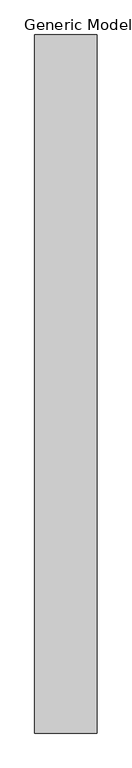
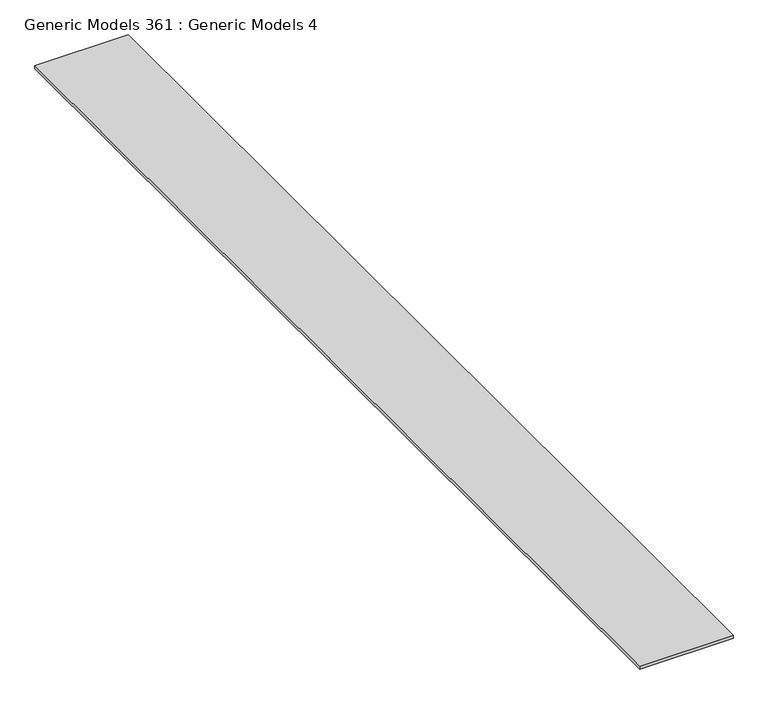
"""IFC4 building model written with IfcOpenShell, lengths in millimetres: proxy geometry, Generic Models 361 : Generic Models 4."""

from ifc_helpers import new_model, si_unit, frame, origin, place, context, project, spatial, polyline, outline, extrude, source, transform, mapped, element, save


def generic_models_361_generic_models_4_672dfefd(model_context):
    return source(origin(), model_context, "Body", "SweptSolid", [
        extrude(outline(polyline([(-6356.5236296, -6864.9230338), (-6928.2116813, -6864.9230338), (-6928.2116813, -464.1230338), (-6356.5236296, -464.1230338), (-6356.5236296, -6864.9230338)])), frame((0.0, 0.0, 127342.646), z_axis=(0.0, 0.0, 1.0), x_axis=(1.0, 0.0, 0.0)), (0.0, 0.0, 1.0), 18.9872466),
    ])


if __name__ == "__main__":
    model = new_model("IFC4")
    model_context = context("Model", 3, world=origin())
    ifc_project = project(units=[si_unit("LENGTHUNIT", "METRE", prefix="MILLI")], contexts=[model_context])
    site = spatial("IfcSite", under=ifc_project)
    building = spatial("IfcBuilding", under=site)
    placement = place(None, origin())
    generic_models_361_generic_models_4_shape = generic_models_361_generic_models_4_672dfefd(model_context)
    element("IfcBuildingElementProxy", 1, Name="Generic Models 361 : Generic Models 4", ObjectType="Generic Models 361 : Generic Models 4", at=placement, inside=building, context=model_context, shape_type="MappedRepresentation", body=[
        mapped(generic_models_361_generic_models_4_shape, transform((0.0, 0.0, 0.0), x_axis=(1.0, 0.0, 0.0), y_axis=(0.0, 1.0, 0.0), z_axis=(0.0, 0.0, 1.0))),
    ])
    save(model, "model.ifc")

# Revit data of these elements
# Element 1 (IfcBuildingElementProxy, "Generic Models 361 : Generic Models 4")
#   Materials on its faces: "_HARDWOOD VENEER PLYWOOD (GRADE B, OR BETTER) - MATCH SOLID TRIM SPECIES"
# Materials
#   "_HARDWOOD VENEER PLYWOOD (GRADE B, OR BETTER) - MATCH SOLID TRIM SPECIES": class "Generic", colour RGB 177 130 114, transparency 0, Cost = 0
